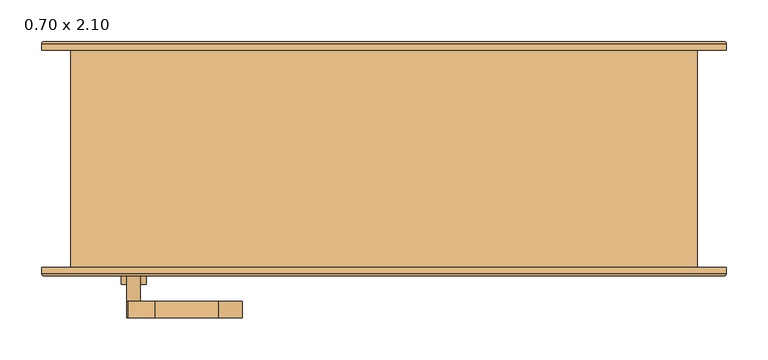
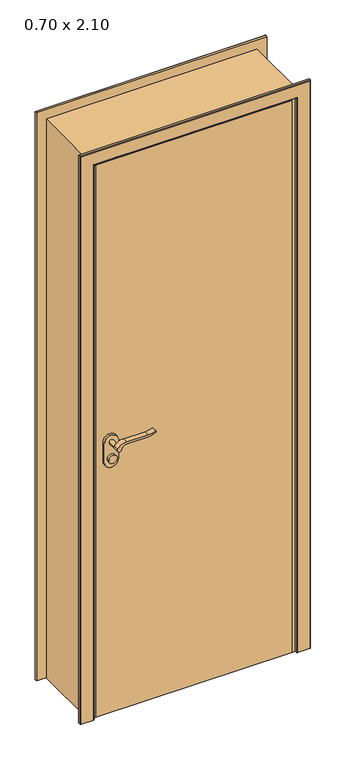
"""IFC4 building model written with IfcOpenShell, lengths in millimetres: door geometry, .CC_ND 300_PORTA SIMPLES DE ABRIR_COM EXTENSÃO : 0.70 x 2.10."""

from ifc_helpers import new_model, si_unit, point, frame, frame_2d, origin, origin_with_axes, place, context, project, spatial, polyline, circle_curve, ellipse_curve, trimmed, segment, composite_curve, outline, extrude, faceted_brep, source, transform, mapped, element, save
from ifc_brep_helpers import plane_surface, cylinder_surface, advanced_brep


def door_0_70_x_2_10_93514c41(model_context):
    return source(origin(), model_context, "Body", "SolidModel", [
        extrude(outline(composite_curve([segment(trimmed(circle_curve(frame_2d((964.5, -300.0)), 15.0), [point((964.5, -285.0))], [point((964.5, -315.0))], False, "CARTESIAN"), True, "CONTINUOUS"), segment(trimmed(circle_curve(frame_2d((964.5, -300.0)), 15.0), [point((964.5, -315.0))], [point((964.5, -285.0))], False, "CARTESIAN"), True, "CONTINUOUS")], self_intersect=False)), frame((0.0, -163.0, 0.0), z_axis=(0.0, 1.0, 0.0), x_axis=(0.0, 0.0, 1.0)), (0.0, 0.0, 1.0), 10.0),
        extrude(outline(composite_curve([segment(trimmed(circle_curve(frame_2d((964.5, -300.0)), 15.0), [point((964.5, -285.0))], [point((964.5, -315.0))], False, "CARTESIAN"), True, "CONTINUOUS"), segment(trimmed(circle_curve(frame_2d((964.5, -300.0)), 15.0), [point((964.5, -315.0))], [point((964.5, -285.0))], False, "CARTESIAN"), True, "CONTINUOUS")], self_intersect=False)), frame((0.0, -103.0, 0.0), z_axis=(0.0, 1.0, 0.0), x_axis=(0.0, 0.0, 1.0)), (0.0, 0.0, 1.0), 10.0),
        extrude(outline(composite_curve([segment(trimmed(circle_curve(frame_2d((1024.5, -300.0)), 8.0), [point((1029.1523287, -306.5081363))], [point((1024.5, -292.0))], False, "CARTESIAN"), True, "CONTINUOUS"), segment(trimmed(circle_curve(frame_2d((1019.3738613, -274.6138099)), 18.1261387), [point((1024.5, -292.0))], [point((1037.5, -274.6138099))], True, "CARTESIAN"), True, "CONTINUOUS"), segment(polyline([(1037.5, -274.6138099), (1037.5, -198.3564091)]), True, "CONTINUOUS"), segment(trimmed(circle_curve(frame_2d((1096.7709207, -201.9396612)), 59.3791355), [point((1037.5, -198.3564091))], [point((1046.7135558, -170.0))], False, "CARTESIAN"), True, "CONTINUOUS"), segment(polyline([(1046.7135558, -170.0), (1049.5, -170.0)]), True, "CONTINUOUS"), segment(trimmed(circle_curve(frame_2d((1127.7850638, -198.4227909)), 83.2850902), [point((1049.5, -170.0))], [point((1044.5, -198.3564091))], True, "CARTESIAN"), True, "CONTINUOUS"), segment(polyline([(1044.5, -198.3564091), (1044.5, -274.6325667)]), True, "CONTINUOUS"), segment(trimmed(circle_curve(frame_2d((1007.2555521, -276.3324871)), 37.2832219), [point((1044.5, -274.6325667))], [point((1029.1523287, -306.5081363))], False, "CARTESIAN"), True, "CONTINUOUS")], self_intersect=False)), frame((0.0, -203.0, 0.0), z_axis=(0.0, 1.0, 0.0), x_axis=(0.0, 0.0, 1.0)), (0.0, 0.0, 1.0), 20.0),
        extrude(outline(composite_curve([segment(trimmed(circle_curve(frame_2d((1019.3738682, -274.6138122)), 18.1261318), [point((1024.4999903, -292.0))], [point((1037.5, -274.6138122))], True, "CARTESIAN"), True, "CONTINUOUS"), segment(polyline([(1037.5, -274.6138122), (1037.5, -198.3564091)]), True, "CONTINUOUS"), segment(trimmed(circle_curve(frame_2d((1096.7709207, -201.9396612)), 59.3791355), [point((1037.5, -198.3564091))], [point((1046.7135558, -170.0))], False, "CARTESIAN"), True, "CONTINUOUS"), segment(polyline([(1046.7135558, -170.0), (1049.5, -170.0)]), True, "CONTINUOUS"), segment(trimmed(circle_curve(frame_2d((1127.7850638, -198.4227909)), 83.2850902), [point((1049.5, -170.0))], [point((1044.5, -198.3564091))], True, "CARTESIAN"), True, "CONTINUOUS"), segment(polyline([(1044.5, -198.3564091), (1044.5, -274.6325667)]), True, "CONTINUOUS"), segment(trimmed(circle_curve(frame_2d((1007.2555521, -276.3324871)), 37.2832219), [point((1044.5, -274.6325667))], [point((1029.1523287, -306.5081363))], False, "CARTESIAN"), True, "CONTINUOUS"), segment(trimmed(circle_curve(frame_2d((1024.5, -300.0)), 8.0), [point((1029.1523287, -306.5081363))], [point((1024.4999903, -292.0))], False, "CARTESIAN"), True, "CONTINUOUS")], self_intersect=False)), frame((0.0, -73.0, 0.0), z_axis=(0.0, 1.0, 0.0), x_axis=(0.0, 0.0, 1.0)), (0.0, 0.0, 1.0), 20.0),
        extrude(outline(composite_curve([segment(trimmed(circle_curve(frame_2d((1024.5, -300.0)), 8.0), [point((1024.5, -292.0))], [point((1024.5, -308.0))], False, "CARTESIAN"), True, "CONTINUOUS"), segment(trimmed(circle_curve(frame_2d((1024.5, -300.0)), 8.0), [point((1024.5, -308.0))], [point((1024.5, -292.0))], False, "CARTESIAN"), True, "CONTINUOUS")], self_intersect=False)), frame((0.0, -183.0, 0.0), z_axis=(0.0, 1.0, 0.0), x_axis=(0.0, 0.0, 1.0)), (0.0, 0.0, 1.0), 30.0),
        extrude(outline(composite_curve([segment(trimmed(circle_curve(frame_2d((1024.5, -300.0)), 8.0), [point((1024.5, -292.0))], [point((1024.5, -308.0))], False, "CARTESIAN"), True, "CONTINUOUS"), segment(trimmed(circle_curve(frame_2d((1024.5, -300.0)), 8.0), [point((1024.5, -308.0))], [point((1024.5, -292.0))], False, "CARTESIAN"), True, "CONTINUOUS")], self_intersect=False)), frame((0.0, -103.0, 0.0), z_axis=(0.0, 1.0, 0.0), x_axis=(0.0, 0.0, 1.0)), (0.0, 0.0, 1.0), 30.0),
        extrude(outline(composite_curve([segment(trimmed(circle_curve(frame_2d((954.5, -300.0)), 25.0), [point((954.5, -325.0))], [point((954.5, -275.0))], False, "CARTESIAN"), True, "CONTINUOUS"), segment(polyline([(954.5, -275.0), (1024.5, -275.0)]), True, "CONTINUOUS"), segment(trimmed(circle_curve(frame_2d((1024.5, -300.0)), 25.0), [point((1024.5, -275.0))], [point((1024.5, -325.0))], False, "CARTESIAN"), True, "CONTINUOUS"), segment(polyline([(1024.5, -325.0), (954.5, -325.0)]), True, "CONTINUOUS")], self_intersect=False)), frame((0.0, -153.0, 0.0), z_axis=(0.0, 1.0, 0.0), x_axis=(0.0, 0.0, 1.0)), (0.0, 0.0, 1.0), 10.0),
        extrude(outline(composite_curve([segment(trimmed(circle_curve(frame_2d((954.5, -300.0)), 25.0), [point((954.5, -325.0))], [point((954.5, -275.0))], False, "CARTESIAN"), True, "CONTINUOUS"), segment(polyline([(954.5, -275.0), (1024.5, -275.0)]), True, "CONTINUOUS"), segment(trimmed(circle_curve(frame_2d((1024.5, -300.0)), 25.0), [point((1024.5, -275.0))], [point((1024.5, -325.0))], False, "CARTESIAN"), True, "CONTINUOUS"), segment(polyline([(1024.5, -325.0), (954.5, -325.0)]), True, "CONTINUOUS")], self_intersect=False)), frame((0.0, -113.0, 0.0), z_axis=(0.0, 1.0, 0.0), x_axis=(0.0, 0.0, 1.0)), (0.0, 0.0, 1.0), 10.0),
        faceted_brep([(342.0, 118.0, 0.0), (375.0, 118.0, 0.0), (375.0, -143.0, 0.0), (350.0, -143.0, 0.0), (350.0, -113.0, 0.0), (342.0, -113.0, 0.0), (342.0, 118.0, 2067.0), (-342.0, 118.0, 2067.0), (-342.0, 118.0, 0.0), (-375.0, 118.0, 0.0), (-375.0, 118.0, 2100.0), (375.0, 118.0, 2100.0), (375.0, -143.0, 2100.0), (-375.0, -143.0, 2100.0), (-375.0, -143.0, 0.0), (-350.0, -143.0, 0.0), (-350.0, -143.0, 2075.0), (350.0, -143.0, 2075.0), (350.0, -113.0, 2075.0), (-350.0, -113.0, 2075.0), (-350.0, -113.0, 0.0), (-342.0, -113.0, 0.0), (-342.0, -113.0, 2067.0), (342.0, -113.0, 2067.0)], [[[0, 1, 2, 3, 4, 5]], [[1, 0, 6, 7, 8, 9, 10, 11]], [[2, 1, 11, 12]], [[3, 2, 12, 13, 14, 15, 16, 17]], [[4, 3, 17, 18]], [[5, 4, 18, 19, 20, 21, 22, 23]], [[0, 5, 23, 6]], [[7, 22, 21, 8]], [[8, 21, 20, 15, 14, 9]], [[13, 10, 9, 14]], [[19, 16, 15, 20]], [[12, 11, 10, 13]], [[18, 17, 16, 19]], [[6, 23, 22, 7]]]),
        extrude(outline(polyline([(-350.0, -113.0), (350.0, -113.0), (350.0, -143.0), (-350.0, -143.0), (-350.0, -113.0)])), origin_with_axes(), (0.0, 0.0, 1.0), 2075.0),
        advanced_brep(
        [(-410.0, -143.0, 0.0), (-360.0, -143.0, 0.0), (-360.0, -150.0, 0.0), (-363.0, -153.0, 0.0), (-407.0, -153.0, 0.0), (-410.0, -150.0, 0.0), (-410.0, -143.0, 2135.0), (410.0, -143.0, 2135.0), (410.0, -143.0, 0.0), (360.0, -143.0, 0.0), (360.0, -143.0, 2085.0), (-360.0, -143.0, 2085.0), (-360.0, -150.0, 2085.0), (-363.0, -153.0, 2088.0), (363.0, -153.0, 2088.0), (363.0, -153.0, 0.0), (407.0, -153.0, 0.0), (407.0, -153.0, 2132.0), (-407.0, -153.0, 2132.0), (-410.0, -150.0, 2135.0), (410.0, -150.0, 2135.0), (410.0, -150.0, 0.0), (360.0, -150.0, 0.0), (360.0, -150.0, 2085.0)],
        [
            (0, 1),
            (1, 2),
            (2, 3, circle_curve(frame((-363.0, -150.0, 0.0), z_axis=(0.0, 0.0, -1.0), x_axis=(1.0, 0.0, 0.0)), 3.0)),
            (3, 4),
            (4, 5, circle_curve(frame((-407.0, -150.0, 0.0), z_axis=(0.0, 0.0, -1.0), x_axis=(1.0, 0.0, 0.0)), 3.0)),
            (5, 0),
            (0, 6),
            (6, 7),
            (7, 8),
            (8, 9),
            (9, 10),
            (10, 11),
            (11, 1),
            (11, 12),
            (12, 2),
            (12, 13, ellipse_curve(frame((-363.0, -150.0, 2088.0), z_axis=(-0.7071067811865475, 0.0, -0.7071067811865475), x_axis=(0.7071067811865474, 0.0, -0.7071067811865476)), 4.2426407, 3.0)),
            (13, 3),
            (13, 14),
            (14, 15),
            (15, 16),
            (16, 17),
            (17, 18),
            (18, 4),
            (18, 19, ellipse_curve(frame((-407.0, -150.0, 2132.0), z_axis=(-0.7071067811865475, 0.0, -0.7071067811865475), x_axis=(0.7071067811865474, 0.0, -0.7071067811865476)), 4.2426407, 3.0)),
            (19, 5),
            (19, 6),
            (7, 20),
            (20, 21),
            (21, 8),
            (21, 16, circle_curve(frame((407.0, -150.0, 0.0), z_axis=(0.0, 0.0, -1.0), x_axis=(-1.0, 0.0, 0.0)), 3.0)),
            (15, 22, circle_curve(frame((363.0, -150.0, 0.0), z_axis=(0.0, 0.0, -1.0), x_axis=(-1.0, 0.0, 0.0)), 3.0)),
            (22, 9),
            (23, 10),
            (22, 23),
            (14, 23, ellipse_curve(frame((363.0, -150.0, 2088.0), z_axis=(0.7071067811865475, 0.0, -0.7071067811865475), x_axis=(0.7071067811865474, 0.0, 0.7071067811865476)), 4.2426407, 3.0)),
            (20, 17, ellipse_curve(frame((407.0, -150.0, 2132.0), z_axis=(0.7071067811865475, 0.0, -0.7071067811865475), x_axis=(0.7071067811865474, 0.0, 0.7071067811865476)), 4.2426407, 3.0)),
            (23, 12),
            (19, 20),
        ],
        [
            plane_surface(frame((-360.0, -143.0, 0.0), z_axis=(0.0, 0.0, -1.0), x_axis=(0.0, 1.0, 0.0))),
            plane_surface(frame((-410.0, -143.0, 0.0), z_axis=(0.0, 1.0, 0.0), x_axis=(0.0, 0.0, 1.0))),
            plane_surface(frame((-360.0, -143.0, 0.0), z_axis=(1.0, 0.0, 0.0), x_axis=(0.0, 0.0, 1.0))),
            cylinder_surface(frame((-363.0, -150.0, 0.0), z_axis=(0.0, 0.0, -1.0), x_axis=(1.0, 0.0, 0.0)), 3.0),
            plane_surface(frame((-363.0, -153.0, 0.0), z_axis=(0.0, -1.0, 0.0), x_axis=(0.0, 0.0, 1.0))),
            cylinder_surface(frame((-407.0, -150.0, 0.0), z_axis=(0.0, 0.0, -1.0), x_axis=(1.0, 0.0, 0.0)), 3.0),
            plane_surface(frame((-410.0, -150.0, 0.0), z_axis=(-1.0, 0.0, 0.0), x_axis=(0.0, 0.0, 1.0))),
            plane_surface(frame((410.0, -150.0, 2135.0), z_axis=(1.0, 0.0, 0.0), x_axis=(0.0, 0.0, -1.0))),
            plane_surface(frame((360.0, -143.0, 0.0), z_axis=(0.0, 0.0, -1.0), x_axis=(0.0, 1.0, 0.0))),
            plane_surface(frame((360.0, -143.0, 2085.0), z_axis=(-1.0, 0.0, 0.0), x_axis=(0.0, 0.0, -1.0))),
            cylinder_surface(frame((363.0, -150.0, 2085.0), z_axis=(0.0, 0.0, 1.0), x_axis=(-1.0, 0.0, 0.0)), 3.0),
            cylinder_surface(frame((407.0, -150.0, 2085.0), z_axis=(0.0, 0.0, 1.0), x_axis=(-1.0, 0.0, 0.0)), 3.0),
            plane_surface(frame((-360.0, -143.0, 2085.0), z_axis=(0.0, 0.0, -1.0), x_axis=(1.0, 0.0, 0.0))),
            plane_surface(frame((-410.0, -150.0, 2135.0), z_axis=(0.0, 0.0, 1.0), x_axis=(1.0, 0.0, 0.0))),
            cylinder_surface(frame((-360.0, -150.0, 2088.0), z_axis=(-1.0, 0.0, 0.0), x_axis=(0.0, 0.0, -1.0)), 3.0),
            cylinder_surface(frame((-360.0, -150.0, 2132.0), z_axis=(-1.0, 0.0, 0.0), x_axis=(0.0, 0.0, -1.0)), 3.0),
        ],
        [
            (0, [[1, 2, 3, 4, 5, 6]]),
            (1, [[-1, 7, 8, 9, 10, 11, 12, 13]]),
            (2, [[-2, -13, 14, 15]]),
            (3, [[-3, -15, 16, 17]]),
            (4, [[-4, -17, 18, 19, 20, 21, 22, 23]]),
            (5, [[-5, -23, 24, 25]]),
            (6, [[-6, -25, 26, -7]]),
            (7, [[27, 28, 29, -9]]),
            (8, [[-29, 30, -20, 31, 32, -10]]),
            (9, [[33, -11, -32, 34]]),
            (10, [[35, -34, -31, -19]]),
            (11, [[36, -21, -30, -28]]),
            (12, [[-14, -12, -33, 37]]),
            (13, [[-26, 38, -27, -8]]),
            (14, [[-16, -37, -35, -18]]),
            (15, [[-24, -22, -36, -38]]),
        ],
    ),
        advanced_brep(
        [(410.0, 118.0, 0.0), (360.0, 118.0, 0.0), (360.0, 125.0157283, 0.0), (362.9842717, 128.0, 0.0), (407.0342217, 128.0, 0.0), (410.0, 125.0342217, 0.0), (410.0, 118.0, 2135.0), (-410.0, 118.0, 2135.0), (-410.0, 118.0, 0.0), (-360.0, 118.0, 0.0), (-360.0, 118.0, 2085.0), (360.0, 118.0, 2085.0), (360.0, 125.0157283, 2085.0), (362.9842717, 128.0, 2087.9842717), (-362.9842717, 128.0, 2087.9842717), (-362.9842717, 128.0, 0.0), (-407.0342217, 128.0, 0.0), (-407.0342217, 128.0, 2132.0342217), (407.0342217, 128.0, 2132.0342217), (410.0, 125.0342217, 2135.0), (-410.0, 125.0342217, 2135.0), (-410.0, 125.0342217, 0.0), (-360.0, 125.0157283, 0.0), (-360.0, 125.0157283, 2085.0)],
        [
            (0, 1),
            (1, 2),
            (2, 3, circle_curve(frame((362.9842717, 125.0157283, 0.0), z_axis=(0.0, 0.0, -1.0), x_axis=(1.0, 0.0, 0.0)), 2.9842717)),
            (3, 4),
            (4, 5, circle_curve(frame((407.0342217, 125.0342217, 0.0), z_axis=(0.0, 0.0, -1.0), x_axis=(1.0, 0.0, 0.0)), 2.9657783)),
            (5, 0),
            (0, 6),
            (6, 7),
            (7, 8),
            (8, 9),
            (9, 10),
            (10, 11),
            (11, 1),
            (11, 12),
            (12, 2),
            (12, 13, ellipse_curve(frame((362.9842717, 125.0157283, 2087.9842717), z_axis=(0.7071067811865475, 0.0, -0.7071067811865475), x_axis=(-0.7071067811865474, 0.0, -0.7071067811865476)), 4.2203975, 2.9842717)),
            (13, 3),
            (13, 14),
            (14, 15),
            (15, 16),
            (16, 17),
            (17, 18),
            (18, 4),
            (18, 19, ellipse_curve(frame((407.0342217, 125.0342217, 2132.0342217), z_axis=(0.7071067811865475, 0.0, -0.7071067811865475), x_axis=(-0.7071067811865474, 0.0, -0.7071067811865476)), 4.1942438, 2.9657783)),
            (19, 5),
            (19, 6),
            (7, 20),
            (20, 21),
            (21, 8),
            (21, 16, circle_curve(frame((-407.0342217, 125.0342217, 0.0), z_axis=(0.0, 0.0, -1.0), x_axis=(-1.0, 0.0, 0.0)), 2.9657783)),
            (15, 22, circle_curve(frame((-362.9842717, 125.0157283, 0.0), z_axis=(0.0, 0.0, -1.0), x_axis=(-1.0, 0.0, 0.0)), 2.9842717)),
            (22, 9),
            (23, 10),
            (22, 23),
            (14, 23, ellipse_curve(frame((-362.9842717, 125.0157283, 2087.9842717), z_axis=(-0.7071067811865475, 0.0, -0.7071067811865475), x_axis=(-0.7071067811865474, 0.0, 0.7071067811865476)), 4.2203975, 2.9842717)),
            (20, 17, ellipse_curve(frame((-407.0342217, 125.0342217, 2132.0342217), z_axis=(-0.7071067811865475, 0.0, -0.7071067811865475), x_axis=(-0.7071067811865474, 0.0, 0.7071067811865476)), 4.1942438, 2.9657783)),
            (23, 12),
            (19, 20),
        ],
        [
            plane_surface(frame((360.0, 118.0, 0.0), z_axis=(0.0, 0.0, -1.0), x_axis=(0.0, 1.0, 0.0))),
            plane_surface(frame((410.0, 118.0, 0.0), z_axis=(0.0, -1.0, 0.0), x_axis=(0.0, 0.0, 1.0))),
            plane_surface(frame((360.0, 118.0, 0.0), z_axis=(-1.0, 0.0, 0.0), x_axis=(0.0, 0.0, 1.0))),
            cylinder_surface(frame((362.9842717, 125.0157283, 0.0), z_axis=(0.0, 0.0, -1.0), x_axis=(1.0, 0.0, 0.0)), 2.9842717),
            plane_surface(frame((362.9842717, 128.0, 0.0), z_axis=(0.0, 1.0, 0.0), x_axis=(0.0, 0.0, 1.0))),
            cylinder_surface(frame((407.0342217, 125.0342217, 0.0), z_axis=(0.0, 0.0, -1.0), x_axis=(1.0, 0.0, 0.0)), 2.9657783),
            plane_surface(frame((410.0, 125.0342217, 0.0), z_axis=(1.0, 0.0, 0.0), x_axis=(0.0, 0.0, 1.0))),
            plane_surface(frame((-410.0, 125.0342217, 2135.0), z_axis=(-1.0, 0.0, 0.0), x_axis=(0.0, 0.0, -1.0))),
            plane_surface(frame((-360.0, 118.0, 0.0), z_axis=(0.0, 0.0, -1.0), x_axis=(0.0, 1.0, 0.0))),
            plane_surface(frame((-360.0, 118.0, 2085.0), z_axis=(1.0, 0.0, 0.0), x_axis=(0.0, 0.0, -1.0))),
            cylinder_surface(frame((-362.9842717, 125.0157283, 2085.0), z_axis=(0.0, 0.0, 1.0), x_axis=(-1.0, 0.0, 0.0)), 2.9842717),
            cylinder_surface(frame((-407.0342217, 125.0342217, 2085.0), z_axis=(0.0, 0.0, 1.0), x_axis=(-1.0, 0.0, 0.0)), 2.9657783),
            plane_surface(frame((360.0, 118.0, 2085.0), z_axis=(0.0, 0.0, -1.0), x_axis=(-1.0, 0.0, 0.0))),
            plane_surface(frame((410.0, 125.0342217, 2135.0), z_axis=(0.0, 0.0, 1.0), x_axis=(-1.0, 0.0, 0.0))),
            cylinder_surface(frame((360.0, 125.0157283, 2087.9842717), z_axis=(1.0, 0.0, 0.0), x_axis=(0.0, 0.0, 1.0)), 2.9842717),
            cylinder_surface(frame((360.0, 125.0342217, 2132.0342217), z_axis=(1.0, 0.0, 0.0), x_axis=(0.0, 0.0, 1.0)), 2.9657783),
        ],
        [
            (0, [[1, 2, 3, 4, 5, 6]]),
            (1, [[-1, 7, 8, 9, 10, 11, 12, 13]]),
            (2, [[-2, -13, 14, 15]]),
            (3, [[-3, -15, 16, 17]]),
            (4, [[-4, -17, 18, 19, 20, 21, 22, 23]]),
            (5, [[-5, -23, 24, 25]]),
            (6, [[-6, -25, 26, -7]]),
            (7, [[27, 28, 29, -9]]),
            (8, [[-29, 30, -20, 31, 32, -10]]),
            (9, [[33, -11, -32, 34]]),
            (10, [[35, -34, -31, -19]]),
            (11, [[36, -21, -30, -28]]),
            (12, [[-14, -12, -33, 37]]),
            (13, [[-26, 38, -27, -8]]),
            (14, [[-16, -37, -35, -18]]),
            (15, [[-24, -22, -36, -38]]),
        ],
    ),
    ])


if __name__ == "__main__":
    model = new_model("IFC4")
    model_context = context("Model", 3, world=origin())
    ifc_project = project(units=[si_unit("LENGTHUNIT", "METRE", prefix="MILLI")], contexts=[model_context])
    site = spatial("IfcSite", under=ifc_project)
    building = spatial("IfcBuilding", under=site)
    placement = place(None, origin())
    door_0_70_x_2_10_shape = door_0_70_x_2_10_93514c41(model_context)
    element("IfcDoor", 1, ObjectType=".CC_ND 300_PORTA SIMPLES DE ABRIR_COM EXTENSÃO : 0.70 x 2.10", at=placement, inside=building, context=model_context, shape_type="MappedRepresentation", body=[
        mapped(door_0_70_x_2_10_shape, transform((0.0, 0.0, 0.0), x_axis=(1.0, 0.0, 0.0), y_axis=(0.0, 1.0, 0.0), z_axis=(0.0, 0.0, 1.0))),
    ])
    save(model, "model.ifc")

# Revit data of these elements
# Type ".CC_ND 300_PORTA SIMPLES DE ABRIR_COM EXTENSÃO : 0.70 x 2.10"
#   Type Mark = "155"
#   Analytic Construction = "<None>"
#   Rough Width = 0.75 m
#   Espessura moldura externa = 0.01 m
#   Espessura moldura interna = 0.01 m
#   Largura moldura = 0.05 m
#   Extensão acabamento exterior [instance default] = 0.00 m
#   Extensão acabamento interior [instance default] = 0.00 m
#   Espessura batente = 0.025 m
#   Thickness = 0.03 m
#   Altura batente = 2.085 m
#   Aux Arco [instance default] = 0.70 m
#   Rough Height = 2.125 m
#   Height = 2.10 m
#   Width = 0.70 m
#   Moldura interna [instance default] = yes
#   Moldura externa [instance default] = yes
#   Porta = .MADEIRA COM PINTURA ESMALTE BRANCO ACETINADO
#   Moldura = .MADEIRA COM PINTURA ESMALTE BRANCO ACETINADO
#   Maçaneta = .ALUMÍNIO
#   Batente = .MADEIRA COM PINTURA ESMALTE BRANCO ACETINADO
#   Function = (empty or 0)
#   Wall Closure = (empty or 0)
# Element 1 (IfcDoor, ".CC_ND 300_PORTA SIMPLES DE ABRIR_COM EXTENSÃO : 0.70 x 2.10")
#   Extensão acabamento interior = 0.025 m
#   Aux Arco = 0.725 m
#   Materials on its faces: ".MADEIRA COM PINTURA ESMALTE BRANCO ACETINADO", ".ALUMÍNIO"
# Materials
#   ".MADEIRA COM PINTURA ESMALTE BRANCO ACETINADO": class ".CC_MADEIRAS", colour RGB 240 240 240, transparency 0, Description = "Madeira com pintura esmalte branco acetinado.", Cost = 0
#   ".ALUMÍNIO": class "CC_METAIS", colour RGB 244 244 244, transparency 0, Description = "Material alumínio", Cost = 0
